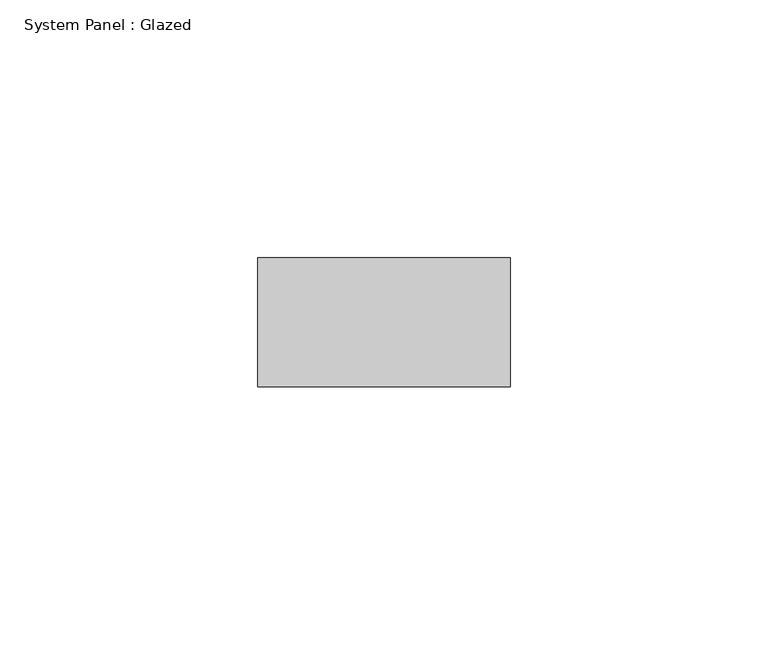
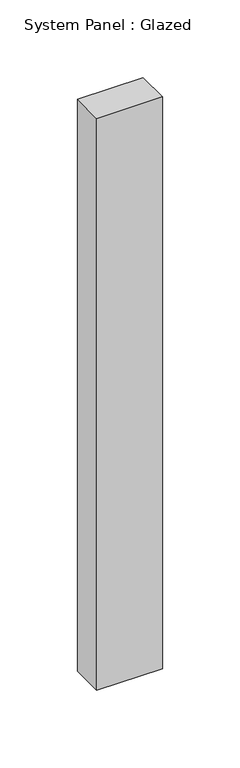
"""IFC4 building model written with IfcOpenShell, lengths in millimetres: plate geometry, System Panel : Glazed."""

import ifcopenshell
import ifcopenshell.guid

model = None  # the IFC model being written
_history = None  # IfcOwnerHistory: only IFC2X3 demands one
_inside = {}  # id of a spatial element -> (the spatial element, [elements in it])
_under = {}  # id of a project, library or spatial element -> (it, [spatial elements below it])
_declared = {}  # id of a project -> (the project, [libraries it declares])
_typed = {}  # id of a type object -> (the type object, [elements of that type])
_made_of = {}  # id of a material, layer set ... -> (it, [elements and type objects made of it])


def new_model(schema):
    """Start an empty IFC model of exactly this schema.

    Asked for "IFC4X3", IfcOpenShell would pick the latest addendum, in which some entities
    have other attributes; the version numbers below select the first issue.
    IFC2X3 requires an IfcOwnerHistory on every rooted entity: one is made here for all.
    """
    global model, _history
    if schema == "IFC4X3":
        model = ifcopenshell.file(schema_version=(4, 3, 0, 0))
    else:
        model = ifcopenshell.file(schema=schema)
    _inside.clear()
    _under.clear()
    _declared.clear()
    _typed.clear()
    _made_of.clear()
    _history = None
    if model.schema == "IFC2X3":
        org = make("IfcOrganization", Name="unknown")
        user = make(
            "IfcPersonAndOrganization",
            ThePerson=make("IfcPerson", FamilyName="unknown"),
            TheOrganization=org,
        )
        app = make(
            "IfcApplication",
            ApplicationDeveloper=org,
            Version="unknown",
            ApplicationFullName="unknown",
            ApplicationIdentifier="unknown",
        )
        _history = make(
            "IfcOwnerHistory",
            OwningUser=user,
            OwningApplication=app,
            ChangeAction="ADDED",
            CreationDate=0,
        )
    return model


def make(cls, **values):
    """One entity of the class cls with the attributes given. An attribute that is None is left unset."""
    return model.create_entity(
        cls, **{name: value for name, value in values.items() if value is not None}
    )


def rooted(cls, **values):
    """An entity with a GlobalId (a new one), such as an element, a storey or a relation."""
    return make(cls, GlobalId=ifcopenshell.guid.new(), OwnerHistory=_history, **values)


def si_unit(unit_type, name, prefix=None):
    """IfcSIUnit, for example si_unit("LENGTHUNIT", "METRE", prefix="MILLI")."""
    return make("IfcSIUnit", UnitType=unit_type, Prefix=prefix, Name=name)


def assignment(units):
    """IfcUnitAssignment: the units of a project."""
    return None if units is None else make("IfcUnitAssignment", Units=units)


def point(xyz):
    """IfcCartesianPoint."""
    return None if xyz is None else make("IfcCartesianPoint", Coordinates=xyz)


def direction(xyz):
    """IfcDirection."""
    return None if xyz is None else make("IfcDirection", DirectionRatios=xyz)


def frame(location, z_axis=None, x_axis=None):
    """IfcAxis2Placement3D, a coordinate frame: its origin and axes. An axis left out is left unset."""
    return make(
        "IfcAxis2Placement3D",
        Location=point(location),
        Axis=direction(z_axis),
        RefDirection=direction(x_axis),
    )


def origin():
    """The frame at (0, 0, 0) with its axes left unset."""
    return frame((0.0, 0.0, 0.0))


def origin_with_axes():
    """The frame at (0, 0, 0) with the z axis (0, 0, 1) and the x axis (1, 0, 0) written out."""
    return frame((0.0, 0.0, 0.0), z_axis=(0.0, 0.0, 1.0), x_axis=(1.0, 0.0, 0.0))


def place(relative_to, where):
    """IfcLocalPlacement: puts the frame where relative to a parent placement (None: the world)."""
    return make(
        "IfcLocalPlacement", PlacementRelTo=relative_to, RelativePlacement=where
    )


def context(
    kind, dimensions, precision=None, world=None, true_north=None, identifier=None
):
    """IfcGeometricRepresentationContext, for example the 3D "Model" context."""
    return make(
        "IfcGeometricRepresentationContext",
        ContextIdentifier=identifier,
        ContextType=kind,
        CoordinateSpaceDimension=dimensions,
        Precision=precision,
        WorldCoordinateSystem=world,
        TrueNorth=true_north,
    )


def project(units=None, contexts=None):
    """IfcProject with its units and contexts."""
    return rooted(
        "IfcProject",
        Name="project",
        RepresentationContexts=contexts,
        UnitsInContext=assignment(units),
    )


def spatial(cls, under=None, at=None, **own):
    """A site, building, storey or space (cls), placed at a placement, below another one or the project."""
    s = rooted(cls, ObjectPlacement=at, **own)
    if under is not None:
        _under.setdefault(under.id(), (under, []))[1].append(s)
    return s


def polyline(points):
    """IfcPolyline through the points."""
    return make("IfcPolyline", Points=[point(p) for p in points])


def outline(outer, holes=None, kind="AREA"):
    """IfcArbitraryClosedProfileDef: a profile drawn as a closed curve; with holes, ...WithVoids."""
    if holes is None:
        return make("IfcArbitraryClosedProfileDef", ProfileType=kind, OuterCurve=outer)
    return make(
        "IfcArbitraryProfileDefWithVoids",
        ProfileType=kind,
        OuterCurve=outer,
        InnerCurves=holes,
    )


def extrude(swept, where, along, depth):
    """IfcExtrudedAreaSolid: the profile swept, set in the frame where, extruded along a direction by depth."""
    return make(
        "IfcExtrudedAreaSolid",
        SweptArea=swept,
        Position=where,
        ExtrudedDirection=direction(along),
        Depth=depth,
    )


def shape(context_of_items, identifier, shape_type, items):
    """IfcShapeRepresentation: the items that make up one representation, for example the "Body"."""
    return make(
        "IfcShapeRepresentation",
        ContextOfItems=context_of_items,
        RepresentationIdentifier=identifier,
        RepresentationType=shape_type,
        Items=items,
    )


def source(mapping_origin, context_of_items, identifier, shape_type, items):
    """IfcRepresentationMap: a shape defined once, which mapped items show again and again."""
    return make(
        "IfcRepresentationMap",
        MappingOrigin=mapping_origin,
        MappedRepresentation=shape(context_of_items, identifier, shape_type, items),
    )


def transform(
    local_origin,
    x_axis=None,
    y_axis=None,
    z_axis=None,
    scale=None,
    scale2=None,
    scale3=None,
    uniform=True,
):
    """IfcCartesianTransformationOperator3D, or its non-uniform kind. x_axis, y_axis, z_axis: its Axis1, 2, 3."""
    if uniform:
        return make(
            "IfcCartesianTransformationOperator3D",
            Axis1=direction(x_axis),
            Axis2=direction(y_axis),
            LocalOrigin=point(local_origin),
            Scale=scale,
            Axis3=direction(z_axis),
        )
    return make(
        "IfcCartesianTransformationOperator3DnonUniform",
        Axis1=direction(x_axis),
        Axis2=direction(y_axis),
        LocalOrigin=point(local_origin),
        Scale=scale,
        Axis3=direction(z_axis),
        Scale2=scale2,
        Scale3=scale3,
    )


def mapped(mapping_source, mapping_target):
    """IfcMappedItem: shows the shape of a source again, moved by a transform."""
    return make(
        "IfcMappedItem", MappingSource=mapping_source, MappingTarget=mapping_target
    )


def made_of(thing, what):
    """Note that an element or type object is made of a material, layer set ...; save() writes the relation."""
    if what is not None:
        _made_of.setdefault(what.id(), (what, []))[1].append(thing)
    return thing


def element(
    cls,
    number,
    at=None,
    inside=None,
    cuts=None,
    type_object=None,
    material=None,
    context=None,
    identifier="Body",
    shape_type=None,
    held_by="IfcProductDefinitionShape",
    body=None,
    shapes=None,
    **own,
):
    """One element of the class cls, such as IfcWall. Its Tag is "e" and its number.

    at: its placement. inside: the storey or other place that contains it. cuts: it is an
    opening in that element (IfcRelVoidsElement). A single representation is given by context,
    identifier, shape_type and body (its items); several are given by shapes. held_by: the class
    of the entity that holds the representations. save() writes the other relations.
    """
    e = rooted(cls, Tag="e%d" % number, ObjectPlacement=at, **own)
    if body is not None:
        shapes = [shape(context, identifier, shape_type, body)]
    if shapes is not None:
        e.Representation = make(held_by, Representations=shapes)
    if inside is not None:
        _inside.setdefault(inside.id(), (inside, []))[1].append(e)
    if cuts is not None:
        rooted(
            "IfcRelVoidsElement", RelatingBuildingElement=cuts, RelatedOpeningElement=e
        )
    if type_object is not None:
        _typed.setdefault(type_object.id(), (type_object, []))[1].append(e)
    return made_of(e, material)


def aggregate(whole, parts):
    """IfcRelAggregates: a whole, such as a stair, and the parts it consists of."""
    return rooted("IfcRelAggregates", RelatingObject=whole, RelatedObjects=parts)


def save(model, path):
    """Write the relations noted so far, then the file.

    IfcRelAggregates (storeys below a building ...), IfcRelContainedInSpatialStructure (elements
    in a storey), IfcRelDefinesByType, IfcRelAssociatesMaterial and IfcRelDeclares: one each for
    every whole, place, type object, material and project.
    """
    for whole, parts in _under.values():
        aggregate(whole, parts)
    for where, things in _inside.values():
        rooted(
            "IfcRelContainedInSpatialStructure",
            RelatedElements=things,
            RelatingStructure=where,
        )
    for kind, things in _typed.values():
        rooted("IfcRelDefinesByType", RelatedObjects=things, RelatingType=kind)
    for what, things in _made_of.values():
        rooted("IfcRelAssociatesMaterial", RelatedObjects=things, RelatingMaterial=what)
    for by, libraries in _declared.values():
        rooted("IfcRelDeclares", RelatingContext=by, RelatedDefinitions=libraries)
    model.write(path)


def system_panel_glazed_455bb06a(model_context):
    return source(origin(), model_context, "Body", "SweptSolid", [
        extrude(outline(polyline([(24.5092572, -49.5), (-24.5092572, -49.5), (-24.5092572, -24.5), (24.5092572, -24.5), (24.5092572, -49.5)])), origin_with_axes(), (0.0, 0.0, 1.0), 450.0),
    ])


if __name__ == "__main__":
    model = new_model("IFC4")
    model_context = context("Model", 3, world=origin())
    ifc_project = project(units=[si_unit("LENGTHUNIT", "METRE", prefix="MILLI")], contexts=[model_context])
    site = spatial("IfcSite", under=ifc_project)
    building = spatial("IfcBuilding", under=site)
    placement = place(None, origin())
    system_panel_glazed_shape = system_panel_glazed_455bb06a(model_context)
    element("IfcPlate", 1, ObjectType="System Panel : Glazed", at=placement, inside=building, context=model_context, shape_type="MappedRepresentation", body=[
        mapped(system_panel_glazed_shape, transform((0.0, 0.0, 0.0), x_axis=(1.0, 0.0, 0.0), y_axis=(0.0, 1.0, 0.0), z_axis=(0.0, 0.0, 1.0))),
    ])
    save(model, "model.ifc")

# Revit data of these elements
# Type "System Panel : Glazed"
#   Keynote = "H11"
#   Construction Type Id = "GSP4R"
#   Analytic Construction = "1/8 in Pilkington single glazing"
#   Visual Light Transmittance = 0.9
#   Solar Heat Gain Coefficient = 0.86
#   Heat Transfer Coefficient (U) = 6.7069 W/(m²·K)
# Element 1 (IfcPlate, "System Panel : Glazed")
#   Materials on its faces: "Glass"
# Materials
#   "Glass": class "Glass", colour RGB 0 128 192, transparency 0.9, Description = "Soda Lime Glass", Cost = 0
